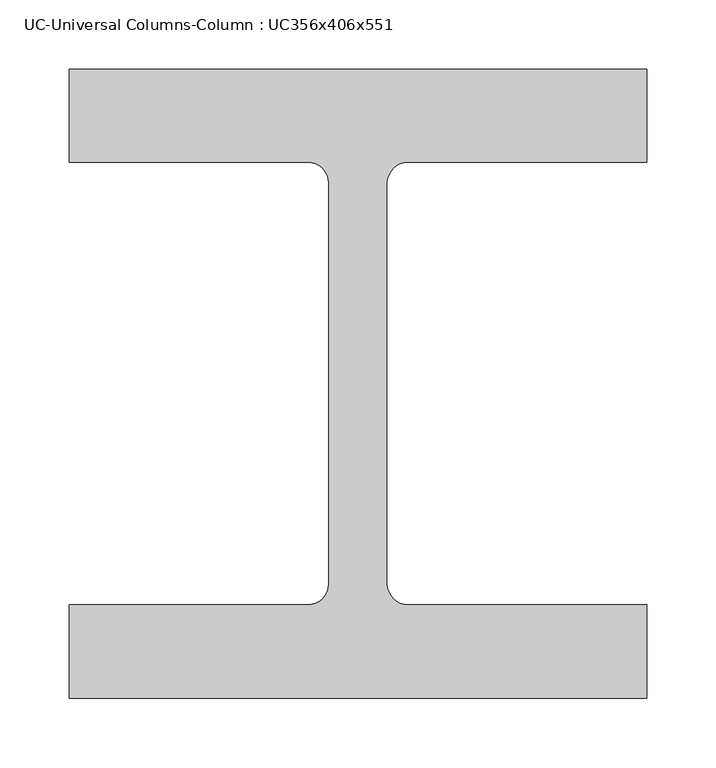
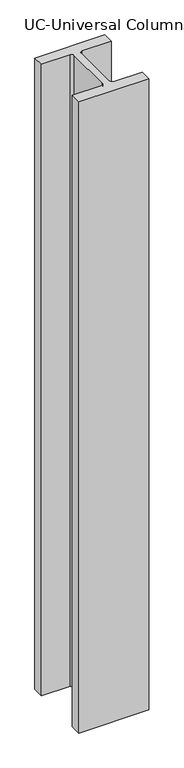
"""IFC4 building model written with IfcOpenShell, lengths in millimetres: column geometry, UC-Universal Columns-Column : UC356x406x551."""

from ifc_helpers import new_model, si_unit, point, frame, frame_2d, origin, place, context, project, spatial, polyline, circle_curve, trimmed, segment, composite_curve, outline, extrude, source, transform, mapped, element, save


def uc_universal_columns_column_uc356x406x551_651137ce(model_context):
    return source(origin(), model_context, "Body", "SweptSolid", [
        extrude(outline(composite_curve([segment(polyline([(209.25, 227.8), (209.25, 160.3), (36.25, 160.3)]), True, "CONTINUOUS"), segment(trimmed(circle_curve(frame_2d((36.25, 145.1)), 15.2), [point((36.25, 160.3))], [point((21.05, 145.1))], True, "CARTESIAN"), True, "CONTINUOUS"), segment(polyline([(21.05, 145.1), (21.05, -145.1)]), True, "CONTINUOUS"), segment(trimmed(circle_curve(frame_2d((36.25, -145.1)), 15.2), [point((21.05, -145.1))], [point((36.25, -160.3))], True, "CARTESIAN"), True, "CONTINUOUS"), segment(polyline([(36.25, -160.3), (209.25, -160.3), (209.25, -227.8), (-209.25, -227.8), (-209.25, -160.3), (-36.25, -160.3)]), True, "CONTINUOUS"), segment(trimmed(circle_curve(frame_2d((-36.25, -145.1)), 15.2), [point((-36.25, -160.3))], [point((-21.05, -145.1))], True, "CARTESIAN"), True, "CONTINUOUS"), segment(polyline([(-21.05, -145.1), (-21.05, 145.1)]), True, "CONTINUOUS"), segment(trimmed(circle_curve(frame_2d((-36.25, 145.1)), 15.2), [point((-21.05, 145.1))], [point((-36.25, 160.3))], True, "CARTESIAN"), True, "CONTINUOUS"), segment(polyline([(-36.25, 160.3), (-209.25, 160.3), (-209.25, 227.8), (209.25, 227.8)]), True, "CONTINUOUS")], self_intersect=False)), frame((0.0, 0.0, 8000.0), z_axis=(0.0, 0.0, 1.0), x_axis=(1.0, 0.0, 0.0)), (0.0, 0.0, 1.0), 4000.0),
    ])


if __name__ == "__main__":
    model = new_model("IFC4")
    model_context = context("Model", 3, world=origin())
    ifc_project = project(units=[si_unit("LENGTHUNIT", "METRE", prefix="MILLI")], contexts=[model_context])
    site = spatial("IfcSite", under=ifc_project)
    building = spatial("IfcBuilding", under=site)
    placement = place(None, origin())
    uc_universal_columns_column_uc356x406x551_shape = uc_universal_columns_column_uc356x406x551_651137ce(model_context)
    element("IfcColumn", 1, ObjectType="UC-Universal Columns-Column : UC356x406x551", at=placement, inside=building, context=model_context, shape_type="MappedRepresentation", body=[
        mapped(uc_universal_columns_column_uc356x406x551_shape, transform((0.0, 0.0, 0.0), x_axis=(1.0, 0.0, 0.0), y_axis=(0.0, 1.0, 0.0), z_axis=(0.0, 0.0, 1.0))),
    ])
    save(model, "model.ifc")

# Revit data of these elements
# Type "UC-Universal Columns-Column : UC356x406x551"
#   Section Name Key = "UC356x406x551"
#   Width = 41.85 cm
#   Web Thickness = 4.21 cm
#   Web Fillet = 1.52 cm
#   Warping Constant = 31100000.0 cm⁶
#   Torsional Moment of Inertia = 9240.00 cm⁴
#   Section Area = 702.0 cm²
#   Plastic Modulus weak axis = 6058.0 cm³
#   Plastic Modulus strong axis = 12076.0 cm³
#   Nominal Weight = 551.00 kgf/m
#   Moment of Inertia weak axis = 82671.00 cm⁴
#   Moment of Inertia strong axis = 226938.00 cm⁴
#   Height = 45.56 cm
#   Flange Thickness = 6.75 cm
#   Elastic Modulus weak axis = 3951.0 cm³
#   Elastic Modulus strong axis = 9962.0 cm³
#   Centroid Vertical = 22.78 cm
#   Centroid Horizontal = 20.925 cm
#   built-in parameter 1005541 = 0.246063 (stored number, unit not read)
#   built-in parameter 1005540 = 0.459318 (stored number, unit not read)
#   Bolt Spacing = 14.0 cm
#   Structural Material [instance default] = Metal - Steel 43-275
#   Type Comments = ""
#   Assembly Code = ""
# Element 1 (IfcColumn, "UC-Universal Columns-Column : UC356x406x551")
#   Materials on its faces: "Metal - Steel 43-275"
# Materials
#   "Metal - Steel 43-275": class "Metal", colour RGB 247 247 247, transparency 0, Cost = 0
